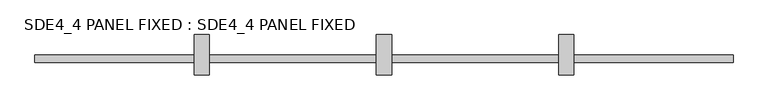
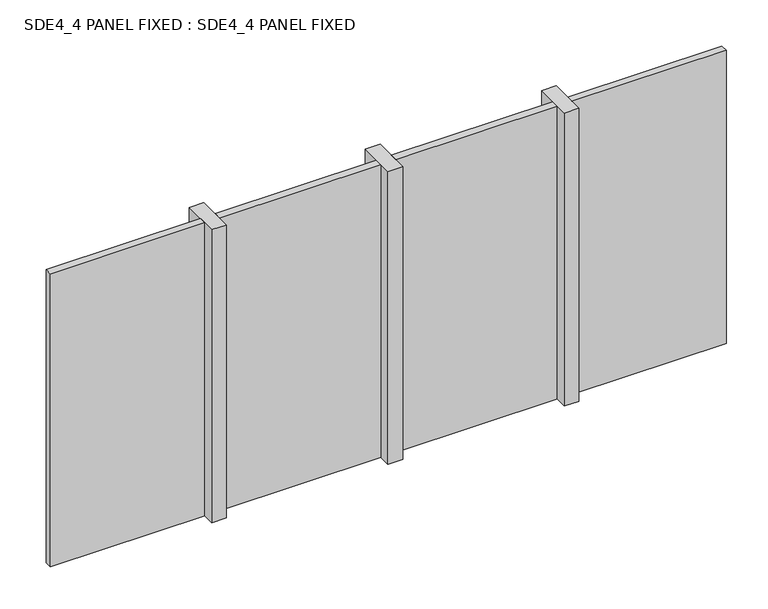
"""IFC4 building model written with IfcOpenShell, lengths in millimetres: plate geometry, SDE4_4 PANEL FIXED : SDE4_4 PANEL FIXED."""

from ifc_helpers import new_model, si_unit, origin, origin_with_axes, place, context, project, spatial, polyline, outline, extrude, source, transform, mapped, element, save


def sde4_4_panel_fixed_sde4_4_panel_fixed_5eb34309(model_context):
    return source(origin(), model_context, "Body", "SweptSolid", [
        extrude(outline(polyline([(-1150.0, -132.5), (-1250.0, -132.5), (-1250.0, 132.5), (-1150.0, 132.5), (-1150.0, -132.5)])), origin_with_axes(), (0.0, 0.0, 1.0), 2110.0),
        extrude(outline(polyline([(50.0, -132.5), (-50.0, -132.5), (-50.0, 132.5), (50.0, 132.5), (50.0, -132.5)])), origin_with_axes(), (0.0, 0.0, 1.0), 2110.0),
        extrude(outline(polyline([(1250.0, -132.5), (1150.0, -132.5), (1150.0, 132.5), (1250.0, 132.5), (1250.0, -132.5)])), origin_with_axes(), (0.0, 0.0, 1.0), 2110.0),
        extrude(outline(polyline([(2299.0, -50.0), (1250.0, -50.0), (1250.0, 0.0), (2299.0, 0.0), (2299.0, -50.0)])), origin_with_axes(), (0.0, 0.0, 1.0), 2110.0),
        extrude(outline(polyline([(1150.0, -50.0), (50.0, -50.0), (50.0, 0.0), (1150.0, 0.0), (1150.0, -50.0)])), origin_with_axes(), (0.0, 0.0, 1.0), 2110.0),
        extrude(outline(polyline([(-50.0, -50.0), (-1150.0, -50.0), (-1150.0, 0.0), (-50.0, 0.0), (-50.0, -50.0)])), origin_with_axes(), (0.0, 0.0, 1.0), 2110.0),
        extrude(outline(polyline([(-1250.0, -50.0), (-2300.0, -50.0), (-2300.0, 0.0), (-1250.0, 0.0), (-1250.0, -50.0)])), origin_with_axes(), (0.0, 0.0, 1.0), 2110.0),
    ])


if __name__ == "__main__":
    model = new_model("IFC4")
    model_context = context("Model", 3, world=origin())
    ifc_project = project(units=[si_unit("LENGTHUNIT", "METRE", prefix="MILLI")], contexts=[model_context])
    site = spatial("IfcSite", under=ifc_project)
    building = spatial("IfcBuilding", under=site)
    placement = place(None, origin())
    sde4_4_panel_fixed_sde4_4_panel_fixed_shape = sde4_4_panel_fixed_sde4_4_panel_fixed_5eb34309(model_context)
    element("IfcPlate", 1, ObjectType="SDE4_4 PANEL FIXED : SDE4_4 PANEL FIXED", at=placement, inside=building, context=model_context, shape_type="MappedRepresentation", body=[
        mapped(sde4_4_panel_fixed_sde4_4_panel_fixed_shape, transform((0.0, 0.0, 0.0), x_axis=(1.0, 0.0, 0.0), y_axis=(0.0, 1.0, 0.0), z_axis=(0.0, 0.0, 1.0))),
    ])
    save(model, "model.ifc")

# Revit data of these elements
# Type "SDE4_4 PANEL FIXED : SDE4_4 PANEL FIXED"
#   Type Mark = "CW-GLASS"
#   Analytic Construction = "<None>"
#   Glass = Glass
#   Frame = Aluminium
# Element 1 (IfcPlate, "SDE4_4 PANEL FIXED : SDE4_4 PANEL FIXED")
#   Materials on its faces: "Glass", "Aluminium"
# Materials
#   "Glass": class "Glass", colour RGB 0 128 192, transparency 0.9, Keynote = "L40", Cost = 0
#   "Aluminium": class "Unassigned", colour RGB 247 247 247, transparency 0, Cost = 0
